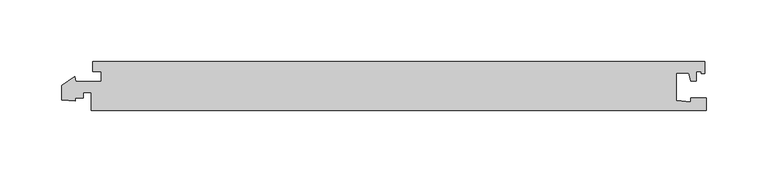
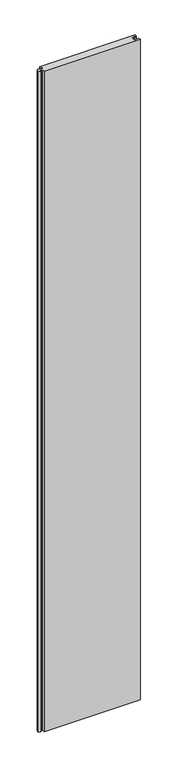
"""IFC4 building model written with IfcOpenShell, lengths in millimetres: proxy geometry, Generic Models 5:Generic Models 5:321804:Generic Models 5:321804 : Generic Models 5:Generic Models 5:321804:26 : Generic Models 5:Generic Models 5:321804:Generic Models 5:321804 : Generic Models 5:Generic Models 5:321804:300761."""

import ifcopenshell
import ifcopenshell.guid

model = None  # the IFC model being written
_history = None  # IfcOwnerHistory: only IFC2X3 demands one
_inside = {}  # id of a spatial element -> (the spatial element, [elements in it])
_under = {}  # id of a project, library or spatial element -> (it, [spatial elements below it])
_declared = {}  # id of a project -> (the project, [libraries it declares])
_typed = {}  # id of a type object -> (the type object, [elements of that type])
_made_of = {}  # id of a material, layer set ... -> (it, [elements and type objects made of it])


def new_model(schema):
    """Start an empty IFC model of exactly this schema.

    Asked for "IFC4X3", IfcOpenShell would pick the latest addendum, in which some entities
    have other attributes; the version numbers below select the first issue.
    IFC2X3 requires an IfcOwnerHistory on every rooted entity: one is made here for all.
    """
    global model, _history
    if schema == "IFC4X3":
        model = ifcopenshell.file(schema_version=(4, 3, 0, 0))
    else:
        model = ifcopenshell.file(schema=schema)
    _inside.clear()
    _under.clear()
    _declared.clear()
    _typed.clear()
    _made_of.clear()
    _history = None
    if model.schema == "IFC2X3":
        org = make("IfcOrganization", Name="unknown")
        user = make(
            "IfcPersonAndOrganization",
            ThePerson=make("IfcPerson", FamilyName="unknown"),
            TheOrganization=org,
        )
        app = make(
            "IfcApplication",
            ApplicationDeveloper=org,
            Version="unknown",
            ApplicationFullName="unknown",
            ApplicationIdentifier="unknown",
        )
        _history = make(
            "IfcOwnerHistory",
            OwningUser=user,
            OwningApplication=app,
            ChangeAction="ADDED",
            CreationDate=0,
        )
    return model


def make(cls, **values):
    """One entity of the class cls with the attributes given. An attribute that is None is left unset."""
    return model.create_entity(
        cls, **{name: value for name, value in values.items() if value is not None}
    )


def rooted(cls, **values):
    """An entity with a GlobalId (a new one), such as an element, a storey or a relation."""
    return make(cls, GlobalId=ifcopenshell.guid.new(), OwnerHistory=_history, **values)


def si_unit(unit_type, name, prefix=None):
    """IfcSIUnit, for example si_unit("LENGTHUNIT", "METRE", prefix="MILLI")."""
    return make("IfcSIUnit", UnitType=unit_type, Prefix=prefix, Name=name)


def assignment(units):
    """IfcUnitAssignment: the units of a project."""
    return None if units is None else make("IfcUnitAssignment", Units=units)


def point(xyz):
    """IfcCartesianPoint."""
    return None if xyz is None else make("IfcCartesianPoint", Coordinates=xyz)


def direction(xyz):
    """IfcDirection."""
    return None if xyz is None else make("IfcDirection", DirectionRatios=xyz)


def frame(location, z_axis=None, x_axis=None):
    """IfcAxis2Placement3D, a coordinate frame: its origin and axes. An axis left out is left unset."""
    return make(
        "IfcAxis2Placement3D",
        Location=point(location),
        Axis=direction(z_axis),
        RefDirection=direction(x_axis),
    )


def origin():
    """The frame at (0, 0, 0) with its axes left unset."""
    return frame((0.0, 0.0, 0.0))


def place(relative_to, where):
    """IfcLocalPlacement: puts the frame where relative to a parent placement (None: the world)."""
    return make(
        "IfcLocalPlacement", PlacementRelTo=relative_to, RelativePlacement=where
    )


def context(
    kind, dimensions, precision=None, world=None, true_north=None, identifier=None
):
    """IfcGeometricRepresentationContext, for example the 3D "Model" context."""
    return make(
        "IfcGeometricRepresentationContext",
        ContextIdentifier=identifier,
        ContextType=kind,
        CoordinateSpaceDimension=dimensions,
        Precision=precision,
        WorldCoordinateSystem=world,
        TrueNorth=true_north,
    )


def project(units=None, contexts=None):
    """IfcProject with its units and contexts."""
    return rooted(
        "IfcProject",
        Name="project",
        RepresentationContexts=contexts,
        UnitsInContext=assignment(units),
    )


def spatial(cls, under=None, at=None, **own):
    """A site, building, storey or space (cls), placed at a placement, below another one or the project."""
    s = rooted(cls, ObjectPlacement=at, **own)
    if under is not None:
        _under.setdefault(under.id(), (under, []))[1].append(s)
    return s


def polyline(points):
    """IfcPolyline through the points."""
    return make("IfcPolyline", Points=[point(p) for p in points])


def outline(outer, holes=None, kind="AREA"):
    """IfcArbitraryClosedProfileDef: a profile drawn as a closed curve; with holes, ...WithVoids."""
    if holes is None:
        return make("IfcArbitraryClosedProfileDef", ProfileType=kind, OuterCurve=outer)
    return make(
        "IfcArbitraryProfileDefWithVoids",
        ProfileType=kind,
        OuterCurve=outer,
        InnerCurves=holes,
    )


def extrude(swept, where, along, depth):
    """IfcExtrudedAreaSolid: the profile swept, set in the frame where, extruded along a direction by depth."""
    return make(
        "IfcExtrudedAreaSolid",
        SweptArea=swept,
        Position=where,
        ExtrudedDirection=direction(along),
        Depth=depth,
    )


def shape(context_of_items, identifier, shape_type, items):
    """IfcShapeRepresentation: the items that make up one representation, for example the "Body"."""
    return make(
        "IfcShapeRepresentation",
        ContextOfItems=context_of_items,
        RepresentationIdentifier=identifier,
        RepresentationType=shape_type,
        Items=items,
    )


def source(mapping_origin, context_of_items, identifier, shape_type, items):
    """IfcRepresentationMap: a shape defined once, which mapped items show again and again."""
    return make(
        "IfcRepresentationMap",
        MappingOrigin=mapping_origin,
        MappedRepresentation=shape(context_of_items, identifier, shape_type, items),
    )


def transform(
    local_origin,
    x_axis=None,
    y_axis=None,
    z_axis=None,
    scale=None,
    scale2=None,
    scale3=None,
    uniform=True,
):
    """IfcCartesianTransformationOperator3D, or its non-uniform kind. x_axis, y_axis, z_axis: its Axis1, 2, 3."""
    if uniform:
        return make(
            "IfcCartesianTransformationOperator3D",
            Axis1=direction(x_axis),
            Axis2=direction(y_axis),
            LocalOrigin=point(local_origin),
            Scale=scale,
            Axis3=direction(z_axis),
        )
    return make(
        "IfcCartesianTransformationOperator3DnonUniform",
        Axis1=direction(x_axis),
        Axis2=direction(y_axis),
        LocalOrigin=point(local_origin),
        Scale=scale,
        Axis3=direction(z_axis),
        Scale2=scale2,
        Scale3=scale3,
    )


def mapped(mapping_source, mapping_target):
    """IfcMappedItem: shows the shape of a source again, moved by a transform."""
    return make(
        "IfcMappedItem", MappingSource=mapping_source, MappingTarget=mapping_target
    )


def made_of(thing, what):
    """Note that an element or type object is made of a material, layer set ...; save() writes the relation."""
    if what is not None:
        _made_of.setdefault(what.id(), (what, []))[1].append(thing)
    return thing


def element(
    cls,
    number,
    at=None,
    inside=None,
    cuts=None,
    type_object=None,
    material=None,
    context=None,
    identifier="Body",
    shape_type=None,
    held_by="IfcProductDefinitionShape",
    body=None,
    shapes=None,
    **own,
):
    """One element of the class cls, such as IfcWall. Its Tag is "e" and its number.

    at: its placement. inside: the storey or other place that contains it. cuts: it is an
    opening in that element (IfcRelVoidsElement). A single representation is given by context,
    identifier, shape_type and body (its items); several are given by shapes. held_by: the class
    of the entity that holds the representations. save() writes the other relations.
    """
    e = rooted(cls, Tag="e%d" % number, ObjectPlacement=at, **own)
    if body is not None:
        shapes = [shape(context, identifier, shape_type, body)]
    if shapes is not None:
        e.Representation = make(held_by, Representations=shapes)
    if inside is not None:
        _inside.setdefault(inside.id(), (inside, []))[1].append(e)
    if cuts is not None:
        rooted(
            "IfcRelVoidsElement", RelatingBuildingElement=cuts, RelatedOpeningElement=e
        )
    if type_object is not None:
        _typed.setdefault(type_object.id(), (type_object, []))[1].append(e)
    return made_of(e, material)


def aggregate(whole, parts):
    """IfcRelAggregates: a whole, such as a stair, and the parts it consists of."""
    return rooted("IfcRelAggregates", RelatingObject=whole, RelatedObjects=parts)


def save(model, path):
    """Write the relations noted so far, then the file.

    IfcRelAggregates (storeys below a building ...), IfcRelContainedInSpatialStructure (elements
    in a storey), IfcRelDefinesByType, IfcRelAssociatesMaterial and IfcRelDeclares: one each for
    every whole, place, type object, material and project.
    """
    for whole, parts in _under.values():
        aggregate(whole, parts)
    for where, things in _inside.values():
        rooted(
            "IfcRelContainedInSpatialStructure",
            RelatedElements=things,
            RelatingStructure=where,
        )
    for kind, things in _typed.values():
        rooted("IfcRelDefinesByType", RelatedObjects=things, RelatingType=kind)
    for what, things in _made_of.values():
        rooted("IfcRelAssociatesMaterial", RelatedObjects=things, RelatingMaterial=what)
    for by, libraries in _declared.values():
        rooted("IfcRelDeclares", RelatingContext=by, RelatedDefinitions=libraries)
    model.write(path)


def generic_models_40f12c52(model_context):
    return source(origin(), model_context, "Body", "SweptSolid", [
        extrude(outline(polyline([(593294.8386129, -568238.0537319), (593284.4802827, -568238.0537319), (593284.4802827, -568260.5495221), (593296.4802827, -568261.5993861), (593296.4802827, -568258.3537319), (593309.2302827, -568258.3537319), (593309.2302827, -568268.5537319), (592809.2302827, -568268.5537319), (592809.2302827, -568254.0537319), (592802.6052827, -568254.0537319), (592802.6052827, -568258.3537319), (592795.9802827, -568258.3537319), (592795.9802827, -568261.0537319), (592784.9802827, -568260.0913566), (592784.9802827, -568248.2332156), (592795.6617846, -568241.1258504), (592796.7142572, -568245.0537319), (592817.4302827, -568245.0537319), (592817.4302827, -568237.0537319), (592810.4802827, -568237.0537319), (592810.4802827, -568228.5537319), (593307.9802827, -568228.5537319), (593307.9802827, -568238.5537319), (593304.9802827, -568238.5537319), (593304.9802827, -568237.0537319), (593301.0302827, -568237.0537319), (593301.0302827, -568244.5537319), (593296.5802827, -568244.5537319), (593294.8386129, -568238.0537319)])), frame((0.0, 0.0, 4883.8301003), z_axis=(0.0, 0.0, 1.0), x_axis=(1.0, 0.0, 0.0)), (0.0, 0.0, 1.0), 3634.8310765),
    ])


if __name__ == "__main__":
    model = new_model("IFC4")
    model_context = context("Model", 3, world=origin())
    ifc_project = project(units=[si_unit("LENGTHUNIT", "METRE", prefix="MILLI")], contexts=[model_context])
    site = spatial("IfcSite", under=ifc_project)
    building = spatial("IfcBuilding", under=site)
    placement = place(None, origin())
    generic_models_shape = generic_models_40f12c52(model_context)
    element("IfcBuildingElementProxy", 1, Name="Generic Models 5:Generic Models 5:321804:Generic Models 5:321804 : Generic Models 5:Generic Models 5:321804:26 : Generic Models 5:Generic Models 5:321804:Generic Models 5:321804 : Generic Models 5:Generic Models 5:321804:300761", ObjectType="Generic Models 5:Generic Models 5:321804:Generic Models 5:321804 : Generic Models 5:Generic Models 5:321804:26 : Generic Models 5:Generic Models 5:321804:Generic Models 5:321804 : Generic Models 5:Generic Models 5:321804:300761", at=placement, inside=building, context=model_context, shape_type="MappedRepresentation", body=[
        mapped(generic_models_shape, transform((0.0, 0.0, 0.0), x_axis=(1.0, 0.0, 0.0), y_axis=(0.0, 1.0, 0.0), z_axis=(0.0, 0.0, 1.0))),
    ])
    save(model, "model.ifc")

# Revit data of these elements
# Type "Generic Models 5:Generic Models 5:321804:Generic Models 5:321804 : Generic Models 5:Generic Models 5:321804:26 : Generic Models 5:Generic Models 5:321804:Generic Models 5:321804 : Generic Models 5:Generic Models 5:321804:300761"
#   NameOverride = "Generic Models 5:Generic Models 5:321804:Generic Models 5:321804 : Generic Models 5:Generic Models 5:321804:300761"
#   ObjectTypeOverride = "Generic Models 5:321804 : Generic Models 5:Generic Models 5:321804"
#   Reference = "Generic Models 5"
#   Tag = "300761"
# Element 1 (IfcBuildingElementProxy, "Generic Models 5:Generic Models 5:321804:Generic Models 5:321804 : Generic Models 5:Generic Models 5:321804:26 : Generic Models 5:Generic Models 5:321804:Generic Models 5:321804 : Generic Models 5:Generic Models 5:321804:300761")
#   Materials on its faces: "POLYCARBONATE PANEL - ARCOPLUS 547"
# Materials
#   "POLYCARBONATE PANEL - ARCOPLUS 547": class "Unassigned", colour RGB 202 225 249, transparency 0.45, Cost = 0
